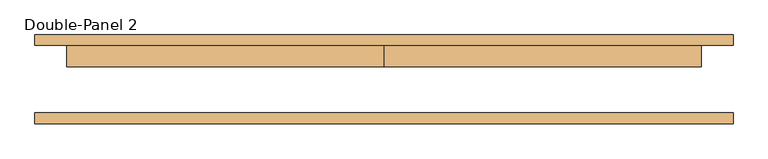
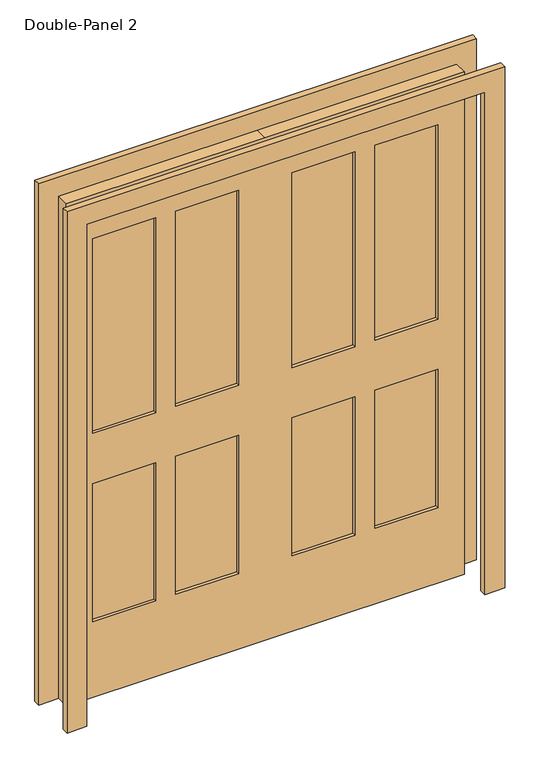
"""IFC4 building model written with IfcOpenShell, lengths in millimetres: door geometry, Double-Panel 2."""

from ifc_helpers import new_model, si_unit, frame, origin, place, context, project, spatial, polyline, outline, extrude, source, transform, mapped, element, save


def double_panel_2_4e97d85f(model_context):
    return source(origin(), model_context, "Body", "SweptSolid", [
        extrude(outline(polyline([(2108.2, -838.2), (0.0, -838.2), (0.0, -762.0), (2032.0, -762.0), (2032.0, 762.0), (0.0, 762.0), (0.0, 838.2), (2108.2, 838.2), (2108.2, -838.2)])), frame((0.0, 80.9625, 0.0), z_axis=(0.0, 1.0, 0.0), x_axis=(0.0, 0.0, 1.0)), (0.0, 0.0, 1.0), 25.4),
        extrude(outline(polyline([(419.1, 68.2625), (660.4, 68.2625), (660.4, 42.8625), (419.1, 42.8625), (419.1, 68.2625)])), frame((0.0, 0.0, 1066.8), z_axis=(0.0, 0.0, 1.0), x_axis=(1.0, 0.0, 0.0)), (0.0, 0.0, 1.0), 787.4),
        extrude(outline(polyline([(101.6, 68.2625), (342.9, 68.2625), (342.9, 42.8625), (101.6, 42.8625), (101.6, 68.2625)])), frame((0.0, 0.0, 1066.8), z_axis=(0.0, 0.0, 1.0), x_axis=(1.0, 0.0, 0.0)), (0.0, 0.0, 1.0), 787.4),
        extrude(outline(polyline([(419.1, 68.2625), (660.4, 68.2625), (660.4, 42.8625), (419.1, 42.8625), (419.1, 68.2625)])), frame((0.0, 0.0, 304.8), z_axis=(0.0, 0.0, 1.0), x_axis=(1.0, 0.0, 0.0)), (0.0, 0.0, 1.0), 558.8),
        extrude(outline(polyline([(101.6, 68.2625), (342.9, 68.2625), (342.9, 42.8625), (101.6, 42.8625), (101.6, 68.2625)])), frame((0.0, 0.0, 304.8), z_axis=(0.0, 0.0, 1.0), x_axis=(1.0, 0.0, 0.0)), (0.0, 0.0, 1.0), 558.8),
        extrude(outline(polyline([(-342.9, 68.2625), (-101.6, 68.2625), (-101.6, 42.8625), (-342.9, 42.8625), (-342.9, 68.2625)])), frame((0.0, 0.0, 1066.8), z_axis=(0.0, 0.0, 1.0), x_axis=(1.0, 0.0, 0.0)), (0.0, 0.0, 1.0), 787.4),
        extrude(outline(polyline([(-660.4, 68.2625), (-419.1, 68.2625), (-419.1, 42.8625), (-660.4, 42.8625), (-660.4, 68.2625)])), frame((0.0, 0.0, 1066.8), z_axis=(0.0, 0.0, 1.0), x_axis=(1.0, 0.0, 0.0)), (0.0, 0.0, 1.0), 787.4),
        extrude(outline(polyline([(-342.9, 68.2625), (-101.6, 68.2625), (-101.6, 42.8625), (-342.9, 42.8625), (-342.9, 68.2625)])), frame((0.0, 0.0, 304.8), z_axis=(0.0, 0.0, 1.0), x_axis=(1.0, 0.0, 0.0)), (0.0, 0.0, 1.0), 558.8),
        extrude(outline(polyline([(-660.4, 68.2625), (-419.1, 68.2625), (-419.1, 42.8625), (-660.4, 42.8625), (-660.4, 68.2625)])), frame((0.0, 0.0, 304.8), z_axis=(0.0, 0.0, 1.0), x_axis=(1.0, 0.0, 0.0)), (0.0, 0.0, 1.0), 558.8),
        extrude(outline(polyline([(2032.0, 0.0), (2032.0, -762.0), (0.0, -762.0), (0.0, 0.0), (0.0, 762.0), (2032.0, 762.0), (2032.0, 0.0)]), holes=[polyline([(1854.2, 419.1), (1854.2, 660.4), (1066.8, 660.4), (1066.8, 419.1), (1854.2, 419.1)]), polyline([(1854.2, 101.6), (1854.2, 342.9), (1066.8, 342.9), (1066.8, 101.6), (1854.2, 101.6)]), polyline([(863.6, 419.1), (863.6, 660.4), (304.8, 660.4), (304.8, 419.1), (863.6, 419.1)]), polyline([(863.6, 101.6), (863.6, 342.9), (304.8, 342.9), (304.8, 101.6), (863.6, 101.6)]), polyline([(1066.8, -342.9), (1854.2, -342.9), (1854.2, -101.6), (1066.8, -101.6), (1066.8, -342.9)]), polyline([(1854.2, -660.4), (1854.2, -419.1), (1066.8, -419.1), (1066.8, -660.4), (1854.2, -660.4)]), polyline([(863.6, -342.9), (863.6, -101.6), (304.8, -101.6), (304.8, -342.9), (863.6, -342.9)]), polyline([(863.6, -660.4), (863.6, -419.1), (304.8, -419.1), (304.8, -660.4), (863.6, -660.4)])]), frame((0.0, 30.1625, 0.0), z_axis=(0.0, 1.0, 0.0), x_axis=(0.0, 0.0, 1.0)), (0.0, 0.0, 1.0), 50.8),
        extrude(outline(polyline([(2032.0, -762.0), (2032.0, 762.0), (0.0, 762.0), (0.0, 838.2), (2108.2, 838.2), (2108.2, -838.2), (0.0, -838.2), (0.0, -762.0), (2032.0, -762.0)])), frame((0.0, -106.3625, 0.0), z_axis=(0.0, 1.0, 0.0), x_axis=(0.0, 0.0, 1.0)), (0.0, 0.0, 1.0), 25.4),
    ])


if __name__ == "__main__":
    model = new_model("IFC4")
    model_context = context("Model", 3, world=origin())
    ifc_project = project(units=[si_unit("LENGTHUNIT", "METRE", prefix="MILLI")], contexts=[model_context])
    site = spatial("IfcSite", under=ifc_project)
    building = spatial("IfcBuilding", under=site)
    placement = place(None, origin())
    double_panel_2_shape = double_panel_2_4e97d85f(model_context)
    element("IfcDoor", 1, ObjectType="Double-Panel 2 : 60\" x 80\"  White", at=placement, inside=building, context=model_context, shape_type="MappedRepresentation", body=[
        mapped(double_panel_2_shape, transform((0.0, 0.0, 0.0), x_axis=(1.0, 0.0, 0.0), y_axis=(0.0, 1.0, 0.0), z_axis=(0.0, 0.0, 1.0))),
    ])
    save(model, "model.ifc")

# Revit data of these elements
# Type "Double-Panel 2 : 60\" x 80\"  White"
#   Type Mark = "85"
#   COBie.Type.CreatedBy = "doug.wood@us.ibm.com"
#   COBie.Type.CreatedOn = "2016-04-14T02:07:24"
#   COBie.Type.Name = "Doors_Double-Panel 2_60\" x 80\"  White_85"
#   COBie.Type.Category = "23-30 10 00 : Doors"
#   COBie.Type.Description = "Double-Panel 2_60\" x 80\"  White"
#   COBie.Type.Manufacturer = ""
#   COBie.Type.ModelNumber = ""
#   Construction Type Id = "MDOOR"
#   Assembly Code = "C1020"
#   Analytic Construction = "Metal"
#   COBie.Type.ReplacementCost = 0
#   Thickness = 0' - 2"
#   Heat Transfer Coefficient (U) = 3.7021 W/(m²·K)
#   Height = 6' - 8"
#   Trim Projection Ext = 0' - 1"
#   Trim Projection Int = 0' - 1"
#   Trim Width = 0' - 3"
#   Width = 5' - 0"
#   COBie.Type = no
#   Door Material = Door - Panel
#   Frame Material = Trim - White
#   Visual Light Transmittance = 0
#   Solar Heat Gain Coefficient = 0
#   Function = (empty or 0)
#   Wall Closure = (empty or 0)
# Element 1 (IfcDoor, "Double-Panel 2 : 60\" x 80\"  White")
#   Materials on its faces: "Door - Panel", "Trim - White"
# Materials
#   "Door - Panel": class "Wood", colour RGB 255 255 255, transparency 0, Cost = 0
#   "Trim - White": class "Wood", colour RGB 255 255 255, transparency 0, Cost = 0
